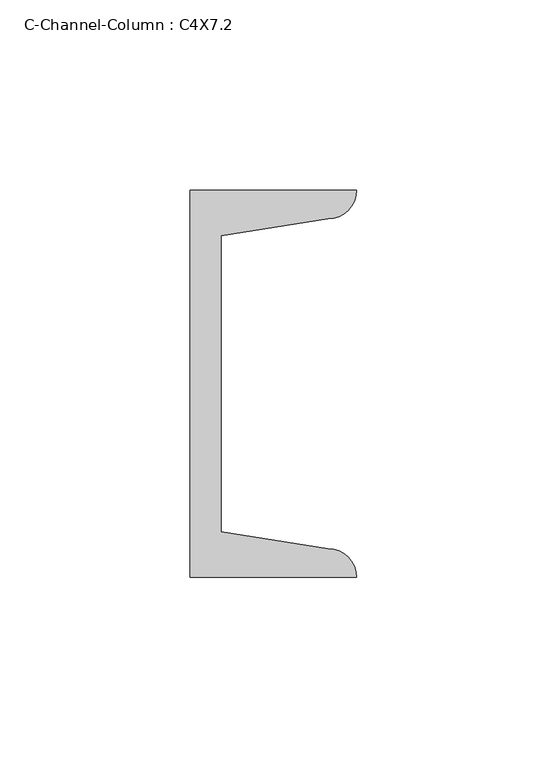
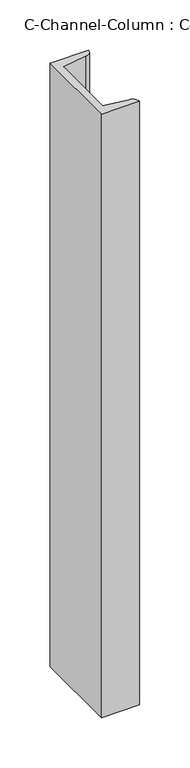
"""IFC4 building model written with IfcOpenShell, lengths in millimetres: column geometry, C-Channel-Column : C4X7.2."""

from ifc_helpers import new_model, si_unit, point, frame, frame_2d, origin, place, context, project, spatial, polyline, circle_curve, trimmed, segment, composite_curve, outline, extrude, source, transform, mapped, element, save


def c_channel_column_c4x7_2_c7b52beb(model_context):
    return source(origin(), model_context, "Body", "SweptSolid", [
        extrude(outline(composite_curve([segment(polyline([(-11.6586, -50.8), (-11.6586, 50.8), (32.0294, 50.8)]), True, "CONTINUOUS"), segment(trimmed(circle_curve(frame_2d((24.511, 50.8)), 7.5184), [point((32.0294, 50.8))], [point((24.511, 43.2816))], False, "CARTESIAN"), True, "CONTINUOUS"), segment(polyline([(24.511, 43.2816), (-3.5052, 38.8442698), (-3.5052, -38.8442698), (24.511, -43.2816)]), True, "CONTINUOUS"), segment(trimmed(circle_curve(frame_2d((24.511, -50.8)), 7.5184), [point((24.511, -43.2816))], [point((32.0294, -50.8))], False, "CARTESIAN"), True, "CONTINUOUS"), segment(polyline([(32.0294, -50.8), (-11.6586, -50.8)]), True, "CONTINUOUS")], self_intersect=False)), frame((0.0, 0.0, 15474.95), z_axis=(0.0, 0.0, 1.0), x_axis=(1.0, 0.0, 0.0)), (0.0, 0.0, 1.0), 730.25),
    ])


if __name__ == "__main__":
    model = new_model("IFC4")
    model_context = context("Model", 3, world=origin())
    ifc_project = project(units=[si_unit("LENGTHUNIT", "METRE", prefix="MILLI")], contexts=[model_context])
    site = spatial("IfcSite", under=ifc_project)
    building = spatial("IfcBuilding", under=site)
    placement = place(None, origin())
    c_channel_column_c4x7_2_shape = c_channel_column_c4x7_2_c7b52beb(model_context)
    element("IfcColumn", 1, ObjectType="C-Channel-Column : C4X7.2", at=placement, inside=building, context=model_context, shape_type="MappedRepresentation", body=[
        mapped(c_channel_column_c4x7_2_shape, transform((0.0, 0.0, 0.0), x_axis=(1.0, 0.0, 0.0), y_axis=(0.0, 1.0, 0.0), z_axis=(0.0, 0.0, 1.0))),
    ])
    save(model, "model.ifc")

# Revit data of these elements
# Type "C-Channel-Column : C4X7.2"
#   Assembly Code = "B10"
#   x = 0' - 0.459"
#   W = 7.2
#   bf = 0' - 1.72"
#   d = 0' - 4"
#   tf = 0' - 0.296"
#   tw = 0' - 0.321"
#   A = 0.0147917 SF
#   Structural Material [instance default] = Steel ASTM A36
# Element 1 (IfcColumn, "C-Channel-Column : C4X7.2")
#   Materials on its faces: "Steel ASTM A36"
# Materials
#   "Steel ASTM A36": class "Metal", colour RGB 199 199 199, transparency 0, Description = "Structural steel, ASTM A36 Grade B, mill finish", Cost = 0
